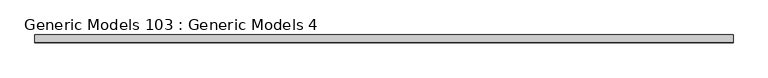
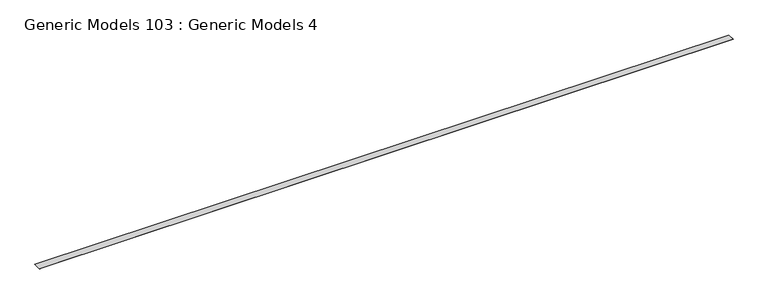
"""IFC4 building model written with IfcOpenShell, lengths in millimetres: proxy geometry, Generic Models 103 : Generic Models 4."""

from ifc_helpers import new_model, si_unit, frame, origin, place, context, project, spatial, polyline, outline, extrude, source, transform, mapped, element, save


def generic_models_103_generic_models_4_3d6319c1(model_context):
    return source(origin(), model_context, "Body", "SweptSolid", [
        extrude(outline(polyline([(7269.7585592, 126937.9496152), (7269.7585592, 126937.1472098), (7056.948377, 126941.5807553), (7056.9649099, 126942.3743331), (7269.7585592, 126937.9496152)])), frame((-10234.5171316, 0.0, 0.0), z_axis=(1.0, 0.0, 0.0), x_axis=(0.0, 1.0, 0.0)), (0.0, 0.0, 1.0), 18643.6),
    ])


if __name__ == "__main__":
    model = new_model("IFC4")
    model_context = context("Model", 3, world=origin())
    ifc_project = project(units=[si_unit("LENGTHUNIT", "METRE", prefix="MILLI")], contexts=[model_context])
    site = spatial("IfcSite", under=ifc_project)
    building = spatial("IfcBuilding", under=site)
    placement = place(None, origin())
    generic_models_103_generic_models_4_shape = generic_models_103_generic_models_4_3d6319c1(model_context)
    element("IfcBuildingElementProxy", 1, Name="Generic Models 103 : Generic Models 4", ObjectType="Generic Models 103 : Generic Models 4", at=placement, inside=building, context=model_context, shape_type="MappedRepresentation", body=[
        mapped(generic_models_103_generic_models_4_shape, transform((0.0, 0.0, 0.0), x_axis=(1.0, 0.0, 0.0), y_axis=(0.0, 1.0, 0.0), z_axis=(0.0, 0.0, 1.0))),
    ])
    save(model, "model.ifc")

# Revit data of these elements
# Element 1 (IfcBuildingElementProxy, "Generic Models 103 : Generic Models 4")
#   Materials on its faces: "_HYDROSTOP LIQUID MEMBRANE - FOLLOW MANU. RECOMMENDED INSTALLATION DETAILS"
# Materials
#   "_HYDROSTOP LIQUID MEMBRANE - FOLLOW MANU. RECOMMENDED INSTALLATION DETAILS": class "Generic", colour RGB 156 184 169, transparency 0, Cost = 0
